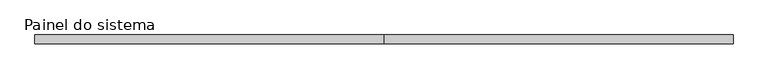
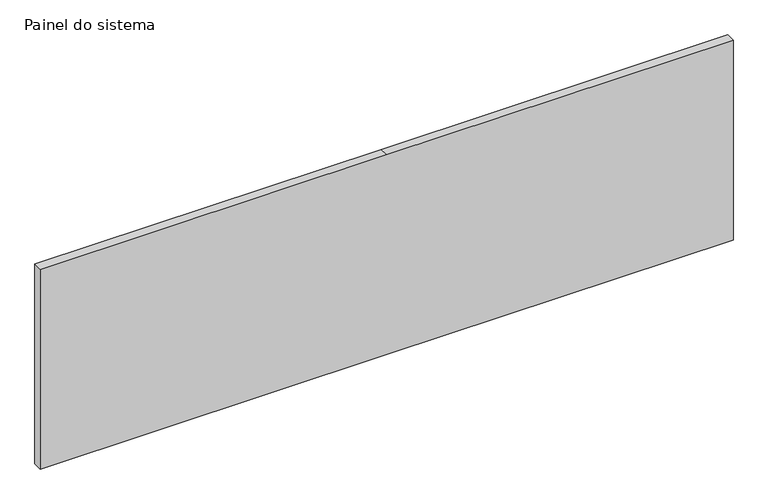
"""IFC4 building model written with IfcOpenShell, lengths in millimetres: plate geometry, Painel do sistema : Envidraçado."""

from ifc_helpers import new_model, si_unit, frame, origin, place, context, project, spatial, polyline, outline, extrude, source, transform, mapped, element, save


def painel_do_sistema_f930648b(model_context):
    return source(origin(), model_context, "Body", "SweptSolid", [
        extrude(outline(polyline([(0.0, -966.7099999), (0.0, 0.0), (0.0, 966.7099999), (590.0, 966.7099999), (590.0, 0.0), (590.0, -966.7099999), (0.0, -966.7099999)])), frame((0.0, -49.5, 0.0), z_axis=(0.0, 1.0, 0.0), x_axis=(0.0, 0.0, 1.0)), (0.0, 0.0, 1.0), 25.0),
    ])


if __name__ == "__main__":
    model = new_model("IFC4")
    model_context = context("Model", 3, world=origin())
    ifc_project = project(units=[si_unit("LENGTHUNIT", "METRE", prefix="MILLI")], contexts=[model_context])
    site = spatial("IfcSite", under=ifc_project)
    building = spatial("IfcBuilding", under=site)
    placement = place(None, origin())
    painel_do_sistema_shape = painel_do_sistema_f930648b(model_context)
    element("IfcPlate", 1, ObjectType="Painel do sistema : Envidraçado", at=placement, inside=building, context=model_context, shape_type="MappedRepresentation", body=[
        mapped(painel_do_sistema_shape, transform((0.0, 0.0, 0.0), x_axis=(1.0, 0.0, 0.0), y_axis=(0.0, 1.0, 0.0), z_axis=(0.0, 0.0, 1.0))),
    ])
    save(model, "model.ifc")

# Revit data of these elements
# Type "Painel do sistema : Envidraçado"
#   Construction Type Id = "GSP4R"
#   Analytic Construction = "Vidraça única Pilkington 1/8 pol"
#   Visual Light Transmittance = 0.9
#   Solar Heat Gain Coefficient = 0.86
#   Heat Transfer Coefficient (U) = 6.7069 W/(m²·K)
# Element 1 (IfcPlate, "Painel do sistema : Envidraçado")
#   Materials on its faces: ".VIDRO GENÉRICO"
# Materials
#   ".VIDRO GENÉRICO": class ".CC_VIDRO", colour RGB 0 128 192, transparency 0.9, Description = "Vidro comum", Cost = 0
